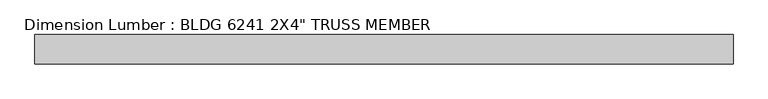
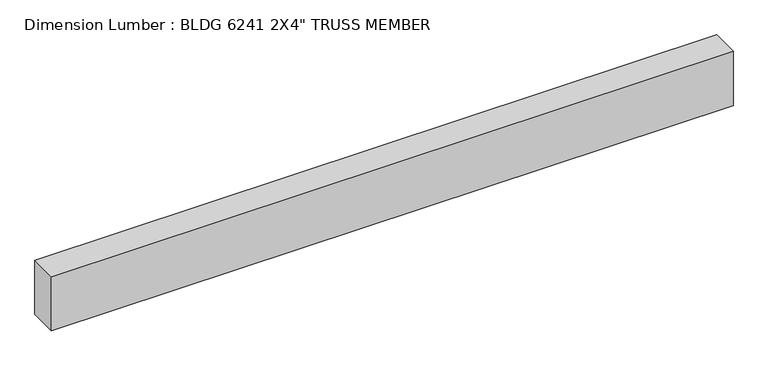
"""IFC4 building model written with IfcOpenShell, lengths in millimetres: beam geometry."""

import ifcopenshell
import ifcopenshell.guid

model = None  # the IFC model being written
_history = None  # IfcOwnerHistory: only IFC2X3 demands one
_inside = {}  # id of a spatial element -> (the spatial element, [elements in it])
_under = {}  # id of a project, library or spatial element -> (it, [spatial elements below it])
_declared = {}  # id of a project -> (the project, [libraries it declares])
_typed = {}  # id of a type object -> (the type object, [elements of that type])
_made_of = {}  # id of a material, layer set ... -> (it, [elements and type objects made of it])


def new_model(schema):
    """Start an empty IFC model of exactly this schema.

    Asked for "IFC4X3", IfcOpenShell would pick the latest addendum, in which some entities
    have other attributes; the version numbers below select the first issue.
    IFC2X3 requires an IfcOwnerHistory on every rooted entity: one is made here for all.
    """
    global model, _history
    if schema == "IFC4X3":
        model = ifcopenshell.file(schema_version=(4, 3, 0, 0))
    else:
        model = ifcopenshell.file(schema=schema)
    _inside.clear()
    _under.clear()
    _declared.clear()
    _typed.clear()
    _made_of.clear()
    _history = None
    if model.schema == "IFC2X3":
        org = make("IfcOrganization", Name="unknown")
        user = make(
            "IfcPersonAndOrganization",
            ThePerson=make("IfcPerson", FamilyName="unknown"),
            TheOrganization=org,
        )
        app = make(
            "IfcApplication",
            ApplicationDeveloper=org,
            Version="unknown",
            ApplicationFullName="unknown",
            ApplicationIdentifier="unknown",
        )
        _history = make(
            "IfcOwnerHistory",
            OwningUser=user,
            OwningApplication=app,
            ChangeAction="ADDED",
            CreationDate=0,
        )
    return model


def make(cls, **values):
    """One entity of the class cls with the attributes given. An attribute that is None is left unset."""
    return model.create_entity(
        cls, **{name: value for name, value in values.items() if value is not None}
    )


def rooted(cls, **values):
    """An entity with a GlobalId (a new one), such as an element, a storey or a relation."""
    return make(cls, GlobalId=ifcopenshell.guid.new(), OwnerHistory=_history, **values)


def si_unit(unit_type, name, prefix=None):
    """IfcSIUnit, for example si_unit("LENGTHUNIT", "METRE", prefix="MILLI")."""
    return make("IfcSIUnit", UnitType=unit_type, Prefix=prefix, Name=name)


def assignment(units):
    """IfcUnitAssignment: the units of a project."""
    return None if units is None else make("IfcUnitAssignment", Units=units)


def point(xyz):
    """IfcCartesianPoint."""
    return None if xyz is None else make("IfcCartesianPoint", Coordinates=xyz)


def direction(xyz):
    """IfcDirection."""
    return None if xyz is None else make("IfcDirection", DirectionRatios=xyz)


def frame(location, z_axis=None, x_axis=None):
    """IfcAxis2Placement3D, a coordinate frame: its origin and axes. An axis left out is left unset."""
    return make(
        "IfcAxis2Placement3D",
        Location=point(location),
        Axis=direction(z_axis),
        RefDirection=direction(x_axis),
    )


def origin():
    """The frame at (0, 0, 0) with its axes left unset."""
    return frame((0.0, 0.0, 0.0))


def place(relative_to, where):
    """IfcLocalPlacement: puts the frame where relative to a parent placement (None: the world)."""
    return make(
        "IfcLocalPlacement", PlacementRelTo=relative_to, RelativePlacement=where
    )


def context(
    kind, dimensions, precision=None, world=None, true_north=None, identifier=None
):
    """IfcGeometricRepresentationContext, for example the 3D "Model" context."""
    return make(
        "IfcGeometricRepresentationContext",
        ContextIdentifier=identifier,
        ContextType=kind,
        CoordinateSpaceDimension=dimensions,
        Precision=precision,
        WorldCoordinateSystem=world,
        TrueNorth=true_north,
    )


def project(units=None, contexts=None):
    """IfcProject with its units and contexts."""
    return rooted(
        "IfcProject",
        Name="project",
        RepresentationContexts=contexts,
        UnitsInContext=assignment(units),
    )


def spatial(cls, under=None, at=None, **own):
    """A site, building, storey or space (cls), placed at a placement, below another one or the project."""
    s = rooted(cls, ObjectPlacement=at, **own)
    if under is not None:
        _under.setdefault(under.id(), (under, []))[1].append(s)
    return s


def polyline(points):
    """IfcPolyline through the points."""
    return make("IfcPolyline", Points=[point(p) for p in points])


def outline(outer, holes=None, kind="AREA"):
    """IfcArbitraryClosedProfileDef: a profile drawn as a closed curve; with holes, ...WithVoids."""
    if holes is None:
        return make("IfcArbitraryClosedProfileDef", ProfileType=kind, OuterCurve=outer)
    return make(
        "IfcArbitraryProfileDefWithVoids",
        ProfileType=kind,
        OuterCurve=outer,
        InnerCurves=holes,
    )


def extrude(swept, where, along, depth):
    """IfcExtrudedAreaSolid: the profile swept, set in the frame where, extruded along a direction by depth."""
    return make(
        "IfcExtrudedAreaSolid",
        SweptArea=swept,
        Position=where,
        ExtrudedDirection=direction(along),
        Depth=depth,
    )


def shape(context_of_items, identifier, shape_type, items):
    """IfcShapeRepresentation: the items that make up one representation, for example the "Body"."""
    return make(
        "IfcShapeRepresentation",
        ContextOfItems=context_of_items,
        RepresentationIdentifier=identifier,
        RepresentationType=shape_type,
        Items=items,
    )


def source(mapping_origin, context_of_items, identifier, shape_type, items):
    """IfcRepresentationMap: a shape defined once, which mapped items show again and again."""
    return make(
        "IfcRepresentationMap",
        MappingOrigin=mapping_origin,
        MappedRepresentation=shape(context_of_items, identifier, shape_type, items),
    )


def transform(
    local_origin,
    x_axis=None,
    y_axis=None,
    z_axis=None,
    scale=None,
    scale2=None,
    scale3=None,
    uniform=True,
):
    """IfcCartesianTransformationOperator3D, or its non-uniform kind. x_axis, y_axis, z_axis: its Axis1, 2, 3."""
    if uniform:
        return make(
            "IfcCartesianTransformationOperator3D",
            Axis1=direction(x_axis),
            Axis2=direction(y_axis),
            LocalOrigin=point(local_origin),
            Scale=scale,
            Axis3=direction(z_axis),
        )
    return make(
        "IfcCartesianTransformationOperator3DnonUniform",
        Axis1=direction(x_axis),
        Axis2=direction(y_axis),
        LocalOrigin=point(local_origin),
        Scale=scale,
        Axis3=direction(z_axis),
        Scale2=scale2,
        Scale3=scale3,
    )


def mapped(mapping_source, mapping_target):
    """IfcMappedItem: shows the shape of a source again, moved by a transform."""
    return make(
        "IfcMappedItem", MappingSource=mapping_source, MappingTarget=mapping_target
    )


def made_of(thing, what):
    """Note that an element or type object is made of a material, layer set ...; save() writes the relation."""
    if what is not None:
        _made_of.setdefault(what.id(), (what, []))[1].append(thing)
    return thing


def element(
    cls,
    number,
    at=None,
    inside=None,
    cuts=None,
    type_object=None,
    material=None,
    context=None,
    identifier="Body",
    shape_type=None,
    held_by="IfcProductDefinitionShape",
    body=None,
    shapes=None,
    **own,
):
    """One element of the class cls, such as IfcWall. Its Tag is "e" and its number.

    at: its placement. inside: the storey or other place that contains it. cuts: it is an
    opening in that element (IfcRelVoidsElement). A single representation is given by context,
    identifier, shape_type and body (its items); several are given by shapes. held_by: the class
    of the entity that holds the representations. save() writes the other relations.
    """
    e = rooted(cls, Tag="e%d" % number, ObjectPlacement=at, **own)
    if body is not None:
        shapes = [shape(context, identifier, shape_type, body)]
    if shapes is not None:
        e.Representation = make(held_by, Representations=shapes)
    if inside is not None:
        _inside.setdefault(inside.id(), (inside, []))[1].append(e)
    if cuts is not None:
        rooted(
            "IfcRelVoidsElement", RelatingBuildingElement=cuts, RelatedOpeningElement=e
        )
    if type_object is not None:
        _typed.setdefault(type_object.id(), (type_object, []))[1].append(e)
    return made_of(e, material)


def aggregate(whole, parts):
    """IfcRelAggregates: a whole, such as a stair, and the parts it consists of."""
    return rooted("IfcRelAggregates", RelatingObject=whole, RelatedObjects=parts)


def save(model, path):
    """Write the relations noted so far, then the file.

    IfcRelAggregates (storeys below a building ...), IfcRelContainedInSpatialStructure (elements
    in a storey), IfcRelDefinesByType, IfcRelAssociatesMaterial and IfcRelDeclares: one each for
    every whole, place, type object, material and project.
    """
    for whole, parts in _under.values():
        aggregate(whole, parts)
    for where, things in _inside.values():
        rooted(
            "IfcRelContainedInSpatialStructure",
            RelatedElements=things,
            RelatingStructure=where,
        )
    for kind, things in _typed.values():
        rooted("IfcRelDefinesByType", RelatedObjects=things, RelatingType=kind)
    for what, things in _made_of.values():
        rooted("IfcRelAssociatesMaterial", RelatedObjects=things, RelatingMaterial=what)
    for by, libraries in _declared.values():
        rooted("IfcRelDeclares", RelatingContext=by, RelatedDefinitions=libraries)
    model.write(path)


def beam_85682148(model_context):
    return source(origin(), model_context, "Body", "SweptSolid", [
        extrude(outline(polyline([(595.8662636, -25.4), (-609.6, -25.4), (-609.6, 25.4), (595.8662636, 25.4), (595.8662636, -25.4)])), frame((0.0, 0.0, -50.8), z_axis=(0.0, 0.0, 1.0), x_axis=(1.0, 0.0, 0.0)), (0.0, 0.0, 1.0), 101.6),
    ])


if __name__ == "__main__":
    model = new_model("IFC4")
    model_context = context("Model", 3, world=origin())
    ifc_project = project(units=[si_unit("LENGTHUNIT", "METRE", prefix="MILLI")], contexts=[model_context])
    site = spatial("IfcSite", under=ifc_project)
    building = spatial("IfcBuilding", under=site)
    placement = place(None, origin())
    beam_shape = beam_85682148(model_context)
    element("IfcBeam", 1, ObjectType="Dimension Lumber : BLDG 6241 2X4\" TRUSS MEMBER", at=placement, inside=building, context=model_context, shape_type="MappedRepresentation", body=[
        mapped(beam_shape, transform((0.0, 0.0, 0.0), x_axis=(1.0, 0.0, 0.0), y_axis=(0.0, 1.0, 0.0), z_axis=(0.0, 0.0, 1.0))),
    ])
    save(model, "model.ifc")

# Revit data of these elements
# Type "Dimension Lumber : BLDG 6241 2X4\" TRUSS MEMBER"
#   Assembly Code = "B10"
#   A = 0.273472 SF
#   Length [instance default] = 5' - 0"
#   b = 0' - 2"
#   d = 0' - 4"
#   Structural Material [instance default] = Softwood, Lumber
# Element 1 (IfcBeam, "Dimension Lumber : BLDG 6241 2X4\" TRUSS MEMBER")
#   Materials on its faces: "Softwood, Lumber"
# Materials
#   "Softwood, Lumber": class "Wood", colour RGB 223 192 134, transparency 0, Description = "Pinus Echinata", Cost = 0
